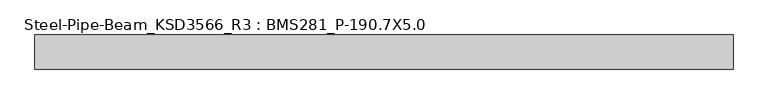
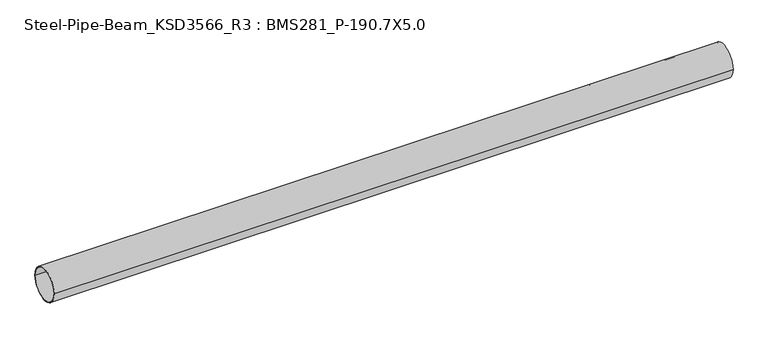
"""IFC4 building model written with IfcOpenShell, lengths in millimetres: member geometry, Steel-Pipe-Beam_KSD3566_R3 : BMS281_P-190.7X5.0."""

from ifc_helpers import new_model, si_unit, point, frame, origin, origin_2d, place, context, project, spatial, circle_curve, trimmed, segment, composite_curve, outline, extrude, source, transform, mapped, element, save


def steel_pipe_beam_ksd3566_r3_bms281_p_190_7x5_0_e615c20f(model_context):
    return source(origin(), model_context, "Body", "SweptSolid", [
        extrude(outline(composite_curve([segment(trimmed(circle_curve(origin_2d(), 95.35), [point((-95.35, 0.0))], [point((95.35, 0.0))], False, "CARTESIAN"), True, "CONTINUOUS"), segment(trimmed(circle_curve(origin_2d(), 95.35), [point((95.35, 0.0))], [point((-95.35, 0.0))], False, "CARTESIAN"), True, "CONTINUOUS")], self_intersect=False), holes=[composite_curve([segment(trimmed(circle_curve(origin_2d(), 90.35), [point((90.35, 0.0))], [point((-90.35, 0.0))], True, "CARTESIAN"), True, "CONTINUOUS"), segment(trimmed(circle_curve(origin_2d(), 90.35), [point((-90.35, 0.0))], [point((90.35, 0.0))], True, "CARTESIAN"), True, "CONTINUOUS")], self_intersect=False)]), frame((-1965.4682703, 0.0, 0.0), z_axis=(1.0, 0.0, 0.0), x_axis=(0.0, 1.0, 0.0)), (0.0, 0.0, 1.0), 3898.3272248),
    ])


if __name__ == "__main__":
    model = new_model("IFC4")
    model_context = context("Model", 3, world=origin())
    ifc_project = project(units=[si_unit("LENGTHUNIT", "METRE", prefix="MILLI")], contexts=[model_context])
    site = spatial("IfcSite", under=ifc_project)
    building = spatial("IfcBuilding", under=site)
    placement = place(None, origin())
    steel_pipe_beam_ksd3566_r3_bms281_p_190_7x5_0_shape = steel_pipe_beam_ksd3566_r3_bms281_p_190_7x5_0_e615c20f(model_context)
    element("IfcMember", 1, ObjectType="Steel-Pipe-Beam_KSD3566_R3 : BMS281_P-190.7X5.0", at=placement, inside=building, context=model_context, shape_type="MappedRepresentation", body=[
        mapped(steel_pipe_beam_ksd3566_r3_bms281_p_190_7x5_0_shape, transform((0.0, 0.0, 0.0), x_axis=(1.0, 0.0, 0.0), y_axis=(0.0, 1.0, 0.0), z_axis=(0.0, 0.0, 1.0))),
    ])
    save(model, "model.ifc")

# Revit data of these elements
# Type "Steel-Pipe-Beam_KSD3566_R3 : BMS281_P-190.7X5.0"
#   Keynote = "P-190.7X5.0"
#   SteelWeight = "Light"
#   t = 0.0050 m
#   Surface Area = 0.599102 m²/m
#   Section Area = 29.1697 cm²
#   Mass per Unit Length = 22.8982 kg/m
#   Length [instance default] = 1.5000 m
#   D = 0.1907 m
#   hec_material4 [instance default] = none
#   hec_material3 [instance default] = none
#   hec_material2 [instance default] = none
#   hec_material1 [instance default] = none
#   Structural Material [instance default] = Steel, 45-345
#   Assembly Code = ""
# Element 1 (IfcMember, "Steel-Pipe-Beam_KSD3566_R3 : BMS281_P-190.7X5.0")
#   Structural Material = none
# Materials
#   "Steel, 45-345": class "Metal", colour RGB 189 187 185, transparency 0, Description = "Steel 345 MPa", Cost = 0
